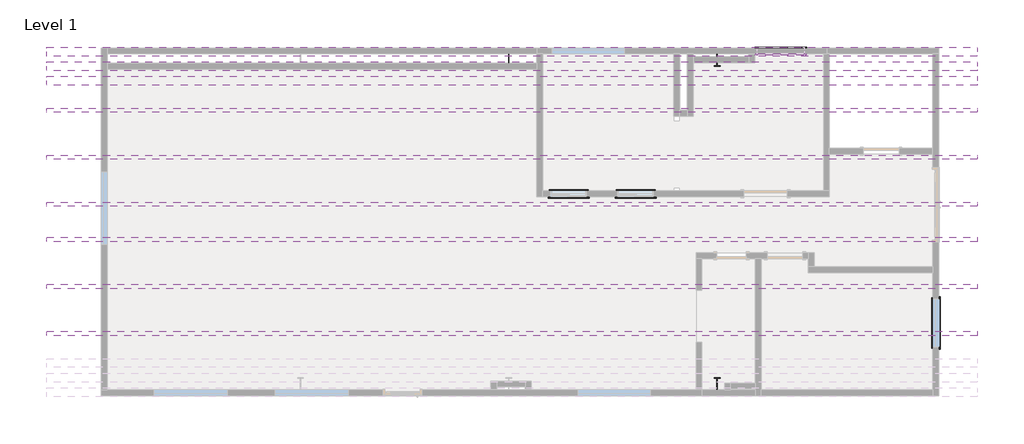
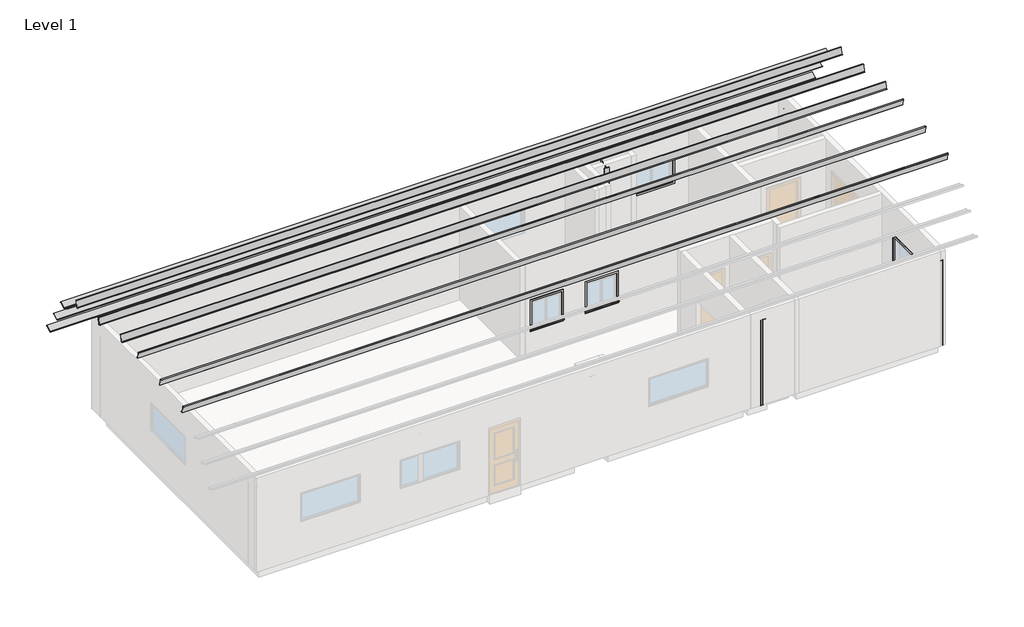
# One storey, part 3 of 3: 9 beams, 8 proxies, 5 columns.
# Revit data of these elements (continued)
# Type "Z Shapes : Z 3X8" (continued)
#   Elastic Modulus strong axis = 0.0193287 (stored number, unit not read)
#   Centroid Vertical = 101.6 mm
#   Centroid Horizontal = 38.1 mm
#   Length [instance default] = 5' - 0"
#   Structural Material [instance default] = Steel ASTM A992
#   Principal Axes Angle = 0
# Type "Trim-Window-Exterior-Flat : with Sill"
#   Trim Width = 0' - 2 1/4"
#   Trim Thickness_Picture Frame = 0' - 1 1/4"
#   Trim Thickness_with Sill = 0' - 0 3/4"
#   Sill Thickness = 0' - 1 1/4"
#   Opening Width [instance default] = 2' - 0"
#   Opening Height [instance default] = 3' - 0"
#   Default Elevation = 4' - 0"
#   Sill = yes
#   Picture Frame = no
#   Trim Material [instance default] = none
# Type "Trim-Window-Interior-Flat : Picture Frame"
#   Trim Thickness_Picture Frame = 0' - 1 1/4"
#   Trim Width = 0' - 2 1/4"
#   Trim Thickness_with Sill = 0' - 0 3/4"
#   Sill Thickness = 0' - 1 1/4"
#   Opening Width [instance default] = 2' - 0"
#   Opening Height [instance default] = 3' - 0"
#   Default Elevation = 4' - 0"
#   Sill = no
#   Picture Frame = yes
#   Trim Material [instance default] = none
# Type "W-Wide Flange-Column : W6X18.5"
#   Assembly Code = "B10"
#   W = 18.5
#   bf = 0' - 6"
#   d = 1' - 6 1/2"
#   k = 0' - 0 7/8"
#   kr = 0' - 0.47"
#   tf = 0' - 0.405"
#   tw = 0' - 0.26"
#   A = 0.0329167 SF
#   Structural Material [instance default] = Steel ASTM A992
# Elements 1, 2, 3, 4, 5, 6, 7, 8, 9 (IfcBeam, "Z Shapes : Z 3X8")
#   Comments = ""
#   Structural Material = Steel ASTM A992
#   Phase Created = New Construction
#   Materials on its faces: "Steel ASTM A992"
# Elements 10, 11 (IfcBuildingElementProxy, "Trim-Window-Exterior-Flat : with Sill")
#   Opening Width = 4' - 0"
#   Opening Height = 3' - 0"
#   Trim Material = Clad - White
#   Phase Created = New Construction
#   Materials on its faces: "Clad - White"
# Elements 12, 13 (IfcBuildingElementProxy, "Trim-Window-Exterior-Flat : with Sill")
#   Opening Width = 3' - 0"
#   Opening Height = 3' - 0"
#   Trim Material = Clad - White
#   Phase Created = New Construction
#   Materials on its faces: "Clad - White"
# Elements 14, 15 (IfcBuildingElementProxy, "Trim-Window-Interior-Flat : Picture Frame")
#   Opening Width = 4' - 0"
#   Opening Height = 3' - 0"
#   Trim Material = Wood - Stained
#   Phase Created = New Construction
#   Materials on its faces: "Wood - Stained"
# Elements 16, 17 (IfcBuildingElementProxy, "Trim-Window-Interior-Flat : Picture Frame")
#   Opening Width = 3' - 0"
#   Opening Height = 3' - 0"
#   Trim Material = Wood - Stained
#   Phase Created = New Construction
#   Materials on its faces: "Wood - Stained"
# Elements 18, 19, 20, 21, 22 (IfcColumn, "W-Wide Flange-Column : W6X18.5")
#   Comments = ""
#   Structural Material = Steel ASTM A992
#   Phase Created = New Construction
#   Materials on its faces: "Steel ASTM A992"
# Materials
#   "Steel ASTM A992": class "Metal", colour RGB 189 187 185, transparency 0, Description = "Structural steel 50ksi", Cost = 0
#   "Clad - White": class "Wood", colour RGB 242 242 238, transparency 0, Cost = 0
#   "Wood - Stained": class "Wood", colour RGB 224 178 126, transparency 0, Cost = 0
